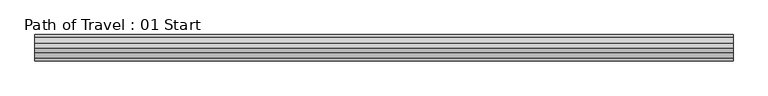
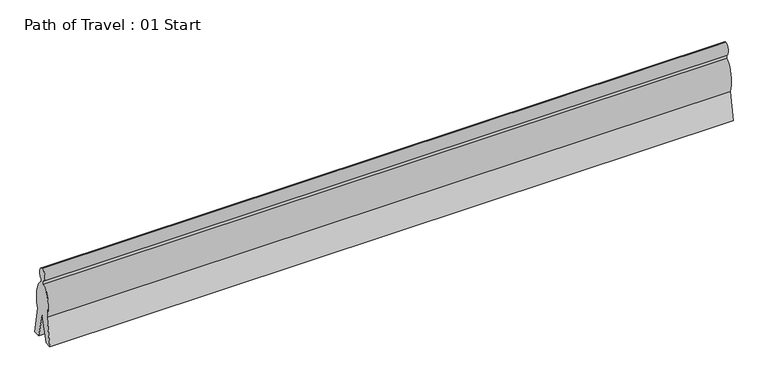
"""IFC4 building model written with IfcOpenShell, lengths in millimetres: proxy geometry, Path of Travel : 01 Start."""

import ifcopenshell
import ifcopenshell.guid

model = None  # the IFC model being written
_history = None  # IfcOwnerHistory: only IFC2X3 demands one
_inside = {}  # id of a spatial element -> (the spatial element, [elements in it])
_under = {}  # id of a project, library or spatial element -> (it, [spatial elements below it])
_declared = {}  # id of a project -> (the project, [libraries it declares])
_typed = {}  # id of a type object -> (the type object, [elements of that type])
_made_of = {}  # id of a material, layer set ... -> (it, [elements and type objects made of it])


def new_model(schema):
    """Start an empty IFC model of exactly this schema.

    Asked for "IFC4X3", IfcOpenShell would pick the latest addendum, in which some entities
    have other attributes; the version numbers below select the first issue.
    IFC2X3 requires an IfcOwnerHistory on every rooted entity: one is made here for all.
    """
    global model, _history
    if schema == "IFC4X3":
        model = ifcopenshell.file(schema_version=(4, 3, 0, 0))
    else:
        model = ifcopenshell.file(schema=schema)
    _inside.clear()
    _under.clear()
    _declared.clear()
    _typed.clear()
    _made_of.clear()
    _history = None
    if model.schema == "IFC2X3":
        org = make("IfcOrganization", Name="unknown")
        user = make(
            "IfcPersonAndOrganization",
            ThePerson=make("IfcPerson", FamilyName="unknown"),
            TheOrganization=org,
        )
        app = make(
            "IfcApplication",
            ApplicationDeveloper=org,
            Version="unknown",
            ApplicationFullName="unknown",
            ApplicationIdentifier="unknown",
        )
        _history = make(
            "IfcOwnerHistory",
            OwningUser=user,
            OwningApplication=app,
            ChangeAction="ADDED",
            CreationDate=0,
        )
    return model


def make(cls, **values):
    """One entity of the class cls with the attributes given. An attribute that is None is left unset."""
    return model.create_entity(
        cls, **{name: value for name, value in values.items() if value is not None}
    )


def rooted(cls, **values):
    """An entity with a GlobalId (a new one), such as an element, a storey or a relation."""
    return make(cls, GlobalId=ifcopenshell.guid.new(), OwnerHistory=_history, **values)


def si_unit(unit_type, name, prefix=None):
    """IfcSIUnit, for example si_unit("LENGTHUNIT", "METRE", prefix="MILLI")."""
    return make("IfcSIUnit", UnitType=unit_type, Prefix=prefix, Name=name)


def assignment(units):
    """IfcUnitAssignment: the units of a project."""
    return None if units is None else make("IfcUnitAssignment", Units=units)


def point(xyz):
    """IfcCartesianPoint."""
    return None if xyz is None else make("IfcCartesianPoint", Coordinates=xyz)


def direction(xyz):
    """IfcDirection."""
    return None if xyz is None else make("IfcDirection", DirectionRatios=xyz)


def frame(location, z_axis=None, x_axis=None):
    """IfcAxis2Placement3D, a coordinate frame: its origin and axes. An axis left out is left unset."""
    return make(
        "IfcAxis2Placement3D",
        Location=point(location),
        Axis=direction(z_axis),
        RefDirection=direction(x_axis),
    )


def origin():
    """The frame at (0, 0, 0) with its axes left unset."""
    return frame((0.0, 0.0, 0.0))


def place(relative_to, where):
    """IfcLocalPlacement: puts the frame where relative to a parent placement (None: the world)."""
    return make(
        "IfcLocalPlacement", PlacementRelTo=relative_to, RelativePlacement=where
    )


def context(
    kind, dimensions, precision=None, world=None, true_north=None, identifier=None
):
    """IfcGeometricRepresentationContext, for example the 3D "Model" context."""
    return make(
        "IfcGeometricRepresentationContext",
        ContextIdentifier=identifier,
        ContextType=kind,
        CoordinateSpaceDimension=dimensions,
        Precision=precision,
        WorldCoordinateSystem=world,
        TrueNorth=true_north,
    )


def project(units=None, contexts=None):
    """IfcProject with its units and contexts."""
    return rooted(
        "IfcProject",
        Name="project",
        RepresentationContexts=contexts,
        UnitsInContext=assignment(units),
    )


def spatial(cls, under=None, at=None, **own):
    """A site, building, storey or space (cls), placed at a placement, below another one or the project."""
    s = rooted(cls, ObjectPlacement=at, **own)
    if under is not None:
        _under.setdefault(under.id(), (under, []))[1].append(s)
    return s


def ellipse_curve(where, semi_axis1, semi_axis2):
    """IfcEllipse in the frame where."""
    return make(
        "IfcEllipse", Position=where, SemiAxis1=semi_axis1, SemiAxis2=semi_axis2
    )


def trimmed(basis, trim1, trim2, sense, master):
    """IfcTrimmedCurve: the piece of a basis curve between two trims."""
    return make(
        "IfcTrimmedCurve",
        BasisCurve=basis,
        Trim1=trim1,
        Trim2=trim2,
        SenseAgreement=sense,
        MasterRepresentation=master,
    )


def shape(context_of_items, identifier, shape_type, items):
    """IfcShapeRepresentation: the items that make up one representation, for example the "Body"."""
    return make(
        "IfcShapeRepresentation",
        ContextOfItems=context_of_items,
        RepresentationIdentifier=identifier,
        RepresentationType=shape_type,
        Items=items,
    )


def source(mapping_origin, context_of_items, identifier, shape_type, items):
    """IfcRepresentationMap: a shape defined once, which mapped items show again and again."""
    return make(
        "IfcRepresentationMap",
        MappingOrigin=mapping_origin,
        MappedRepresentation=shape(context_of_items, identifier, shape_type, items),
    )


def transform(
    local_origin,
    x_axis=None,
    y_axis=None,
    z_axis=None,
    scale=None,
    scale2=None,
    scale3=None,
    uniform=True,
):
    """IfcCartesianTransformationOperator3D, or its non-uniform kind. x_axis, y_axis, z_axis: its Axis1, 2, 3."""
    if uniform:
        return make(
            "IfcCartesianTransformationOperator3D",
            Axis1=direction(x_axis),
            Axis2=direction(y_axis),
            LocalOrigin=point(local_origin),
            Scale=scale,
            Axis3=direction(z_axis),
        )
    return make(
        "IfcCartesianTransformationOperator3DnonUniform",
        Axis1=direction(x_axis),
        Axis2=direction(y_axis),
        LocalOrigin=point(local_origin),
        Scale=scale,
        Axis3=direction(z_axis),
        Scale2=scale2,
        Scale3=scale3,
    )


def mapped(mapping_source, mapping_target):
    """IfcMappedItem: shows the shape of a source again, moved by a transform."""
    return make(
        "IfcMappedItem", MappingSource=mapping_source, MappingTarget=mapping_target
    )


def made_of(thing, what):
    """Note that an element or type object is made of a material, layer set ...; save() writes the relation."""
    if what is not None:
        _made_of.setdefault(what.id(), (what, []))[1].append(thing)
    return thing


def element(
    cls,
    number,
    at=None,
    inside=None,
    cuts=None,
    type_object=None,
    material=None,
    context=None,
    identifier="Body",
    shape_type=None,
    held_by="IfcProductDefinitionShape",
    body=None,
    shapes=None,
    **own,
):
    """One element of the class cls, such as IfcWall. Its Tag is "e" and its number.

    at: its placement. inside: the storey or other place that contains it. cuts: it is an
    opening in that element (IfcRelVoidsElement). A single representation is given by context,
    identifier, shape_type and body (its items); several are given by shapes. held_by: the class
    of the entity that holds the representations. save() writes the other relations.
    """
    e = rooted(cls, Tag="e%d" % number, ObjectPlacement=at, **own)
    if body is not None:
        shapes = [shape(context, identifier, shape_type, body)]
    if shapes is not None:
        e.Representation = make(held_by, Representations=shapes)
    if inside is not None:
        _inside.setdefault(inside.id(), (inside, []))[1].append(e)
    if cuts is not None:
        rooted(
            "IfcRelVoidsElement", RelatingBuildingElement=cuts, RelatedOpeningElement=e
        )
    if type_object is not None:
        _typed.setdefault(type_object.id(), (type_object, []))[1].append(e)
    return made_of(e, material)


def aggregate(whole, parts):
    """IfcRelAggregates: a whole, such as a stair, and the parts it consists of."""
    return rooted("IfcRelAggregates", RelatingObject=whole, RelatedObjects=parts)


def save(model, path):
    """Write the relations noted so far, then the file.

    IfcRelAggregates (storeys below a building ...), IfcRelContainedInSpatialStructure (elements
    in a storey), IfcRelDefinesByType, IfcRelAssociatesMaterial and IfcRelDeclares: one each for
    every whole, place, type object, material and project.
    """
    for whole, parts in _under.values():
        aggregate(whole, parts)
    for where, things in _inside.values():
        rooted(
            "IfcRelContainedInSpatialStructure",
            RelatedElements=things,
            RelatingStructure=where,
        )
    for kind, things in _typed.values():
        rooted("IfcRelDefinesByType", RelatedObjects=things, RelatingType=kind)
    for what, things in _made_of.values():
        rooted("IfcRelAssociatesMaterial", RelatedObjects=things, RelatingMaterial=what)
    for by, libraries in _declared.values():
        rooted("IfcRelDeclares", RelatingContext=by, RelatedDefinitions=libraries)
    model.write(path)


def plane_surface(at):
    """IfcPlane: the flat surface through the origin of the frame at, square to its z axis."""
    return make("IfcPlane", Position=at)


def extruded_surface(curve, direction_of_extrusion, depth):
    """IfcSurfaceOfLinearExtrusion: the curve pushed along a direction by depth."""
    return make(
        "IfcSurfaceOfLinearExtrusion",
        SweptCurve=make("IfcArbitraryOpenProfileDef", ProfileType="CURVE", Curve=curve),
        ExtrudedDirection=direction(direction_of_extrusion),
        Depth=depth,
    )


def advanced_brep(points, edges, surfaces, faces):
    """IfcAdvancedBrep: a solid bounded by faces that lie on surfaces and meet in shared edges.

    An edge is (start, end): straight between two places in points (the first is 0);
    or (start, end, curve); or (start, end, curve, False) where it runs against its curve.
    A face is (place in surfaces, loops), or (place, loops, False) where it looks against
    its surface's normal. A loop lists edges by number (the first is 1), with a minus sign
    where the edge is run from its end to its start. The first loop is the outer one.
    """
    corners = [point(p) for p in points]
    vertices = [make("IfcVertexPoint", VertexGeometry=c) for c in corners]
    made = []
    for start, end, *more in edges:
        made.append(
            make(
                "IfcEdgeCurve",
                EdgeStart=vertices[start],
                EdgeEnd=vertices[end],
                EdgeGeometry=more[0] if more else make("IfcPolyline", Points=[corners[start], corners[end]]),
                SameSense=more[1] if len(more) > 1 else True,
            )
        )
    hull = []
    for where, loops, *sense in faces:
        bounds = []
        for j, loop in enumerate(loops):
            ring = [make("IfcOrientedEdge", EdgeElement=made[abs(k) - 1], Orientation=k > 0) for k in loop]
            bounds.append(
                make(
                    "IfcFaceOuterBound" if j == 0 else "IfcFaceBound",
                    Bound=make("IfcEdgeLoop", EdgeList=ring),
                    Orientation=True,
                )
            )
        hull.append(make("IfcAdvancedFace", Bounds=bounds, FaceSurface=surfaces[where], SameSense=sense[0] if sense else True))
    return make("IfcAdvancedBrep", Outer=make("IfcClosedShell", CfsFaces=hull))


def path_of_travel_01_start_b18a8849(model_context):
    return source(origin(), model_context, "Body", "AdvancedBrep", [
        advanced_brep(
        [(227.5554837, 0.0, 1727.2), (227.5554837, 42.9018657, 1436.6534209), (227.5554837, 42.9018657, 1363.4763406), (227.5554837, 184.1186263, 643.4144547), (227.5554837, 297.5699544, 0.0), (227.5554837, 145.6574193, 0.0), (227.5554837, 0.0, 584.2), (227.5554837, -145.6574193, 0.0), (227.5554837, -297.5699544, 0.0), (227.5554837, -184.1186263, 643.4144547), (227.5554837, -42.9018657, 1363.4763406), (227.5554837, -42.9018657, 1436.6534209), (15924.7554837, 0.0, 1727.2), (15924.7554837, -42.9018657, 1436.6534209), (15924.7554837, -42.9018657, 1363.4763406), (15924.7554837, -184.1186263, 643.4144547), (15924.7554837, -297.5699544, 0.0), (15924.7554837, -145.6574193, 0.0), (15924.7554837, 0.0, 584.2), (15924.7554837, 145.6574193, 0.0), (15924.7554837, 297.5699544, 0.0), (15924.7554837, 184.1186263, 643.4144547), (15924.7554837, 42.9018657, 1363.4763406), (15924.7554837, 42.9018657, 1436.6534209)],
        [
            (0, 1, ellipse_curve(frame((227.5554837, 0.0, 1574.8), z_axis=(-1.0, 0.0, 0.0), x_axis=(0.0, 0.0, 1.0)), 152.4, 101.6)),
            (1, 2),
            (2, 3, ellipse_curve(frame((227.5554837, 0.0, 914.4), z_axis=(-1.0, 0.0, 0.0), x_axis=(0.0, 0.0, -1.0)), 457.2, 228.6)),
            (3, 4),
            (4, 5),
            (5, 6),
            (6, 7),
            (7, 8),
            (8, 9),
            (9, 10, ellipse_curve(frame((227.5554837, 0.0, 914.4), z_axis=(-1.0, 0.0, 0.0), x_axis=(0.0, 0.0, -1.0)), 457.2, 228.6)),
            (10, 11),
            (11, 0, ellipse_curve(frame((227.5554837, 0.0, 1574.8), z_axis=(-1.0, 0.0, 0.0), x_axis=(0.0, 0.0, 1.0)), 152.4, 101.6)),
            (12, 13, ellipse_curve(frame((15924.7554837, 0.0, 1574.8), z_axis=(1.0, 0.0, 0.0), x_axis=(0.0, 0.0, 1.0)), 152.4, 101.6)),
            (13, 14),
            (14, 15, ellipse_curve(frame((15924.7554837, 0.0, 914.4), z_axis=(1.0, 0.0, 0.0), x_axis=(0.0, 0.0, -1.0)), 457.2, 228.6)),
            (15, 16),
            (16, 17),
            (17, 18),
            (18, 19),
            (19, 20),
            (20, 21),
            (21, 22, ellipse_curve(frame((15924.7554837, 0.0, 914.4), z_axis=(1.0, 0.0, 0.0), x_axis=(0.0, 0.0, -1.0)), 457.2, 228.6)),
            (22, 23),
            (23, 12, ellipse_curve(frame((15924.7554837, 0.0, 1574.8), z_axis=(1.0, 0.0, 0.0), x_axis=(0.0, 0.0, 1.0)), 152.4, 101.6)),
            (0, 12),
            (23, 1),
            (22, 2),
            (21, 3),
            (20, 4),
            (19, 5),
            (18, 6),
            (17, 7),
            (16, 8),
            (15, 9),
            (14, 10),
            (13, 11),
        ],
        [
            plane_surface(frame((227.5554837, 0.0, 0.0), z_axis=(-1.0, 0.0, 0.0), x_axis=(0.0, 0.0, 1.0))),
            plane_surface(frame((15924.7554837, 0.0, 0.0), z_axis=(1.0, 0.0, 0.0), x_axis=(0.0, 0.0, 1.0))),
            extruded_surface(trimmed(ellipse_curve(frame((15924.7554837, 0.0, 1574.8), z_axis=(-1.0, 0.0, 0.0), x_axis=(0.0, 0.0, 1.0)), 152.4, 101.6), [point((15924.7554837, 0.0, 1727.2))], [point((15924.7554837, 42.9018657, 1436.6534209))], True, "CARTESIAN"), (-15697.2, 0.0, 0.0), 15697.2),
            plane_surface(frame((227.5554837, 42.9018657, 1436.6534209), z_axis=(0.0, 1.0, 0.0), x_axis=(1.0, 0.0, 0.0))),
            extruded_surface(trimmed(ellipse_curve(frame((15924.7554837, 0.0, 914.4), z_axis=(-1.0, 0.0, 0.0), x_axis=(0.0, 0.0, -1.0)), 457.2, 228.6), [point((15924.7554837, 42.9018657, 1363.4763406))], [point((15924.7554837, 184.1186263, 643.4144547))], True, "CARTESIAN"), (-15697.2, 0.0, 0.0), 15697.2),
            plane_surface(frame((227.5554837, 184.1186263, 643.4144547), z_axis=(0.0, 0.9848077530122078, 0.17364817766693205), x_axis=(1.0, 0.0, 0.0))),
            plane_surface(frame((227.5554837, 297.5699544, 0.0), z_axis=(0.0, 0.0, -1.0), x_axis=(1.0, 0.0, 0.0))),
            plane_surface(frame((227.5554837, 145.6574193, 0.0), z_axis=(0.0, -0.9702957262760199, -0.2419218955995739), x_axis=(1.0, 0.0, 0.0))),
            plane_surface(frame((227.5554837, 0.0, 584.2), z_axis=(0.0, 0.9702957262759961, -0.24192189559966923), x_axis=(1.0, 0.0, 0.0))),
            plane_surface(frame((227.5554837, -145.6574193, 0.0), z_axis=(0.0, 0.0, -1.0), x_axis=(1.0, 0.0, 0.0))),
            plane_surface(frame((227.5554837, -297.5699544, 0.0), z_axis=(0.0, -0.984807753012208, 0.17364817766693066), x_axis=(1.0, 0.0, 0.0))),
            extruded_surface(trimmed(ellipse_curve(frame((15924.7554837, 0.0, 914.4), z_axis=(-1.0, 0.0, 0.0), x_axis=(0.0, 0.0, -1.0)), 457.2, 228.6), [point((15924.7554837, -184.1186263, 643.4144547))], [point((15924.7554837, -42.9018657, 1363.4763406))], True, "CARTESIAN"), (-15697.2, 0.0, 0.0), 15697.2),
            plane_surface(frame((227.5554837, -42.9018657, 1363.4763406), z_axis=(0.0, -1.0, 0.0), x_axis=(1.0, 0.0, 0.0))),
            extruded_surface(trimmed(ellipse_curve(frame((15924.7554837, 0.0, 1574.8), z_axis=(-1.0, 0.0, 0.0), x_axis=(0.0, 0.0, 1.0)), 152.4, 101.6), [point((15924.7554837, -42.9018657, 1436.6534209))], [point((15924.7554837, 0.0, 1727.2))], True, "CARTESIAN"), (-15697.2, 0.0, 0.0), 15697.2),
        ],
        [
            (0, [[1, 2, 3, 4, 5, 6, 7, 8, 9, 10, 11, 12]]),
            (1, [[13, 14, 15, 16, 17, 18, 19, 20, 21, 22, 23, 24]]),
            (2, [[-1, 25, -24, 26]]),
            (3, [[-2, -26, -23, 27]]),
            (4, [[-3, -27, -22, 28]]),
            (5, [[-4, -28, -21, 29]]),
            (6, [[-5, -29, -20, 30]]),
            (7, [[-6, -30, -19, 31]]),
            (8, [[-7, -31, -18, 32]]),
            (9, [[-8, -32, -17, 33]]),
            (10, [[-9, -33, -16, 34]]),
            (11, [[-10, -34, -15, 35]]),
            (12, [[-11, -35, -14, 36]]),
            (13, [[-12, -36, -13, -25]]),
        ],
    ),
    ])


if __name__ == "__main__":
    model = new_model("IFC4")
    model_context = context("Model", 3, world=origin())
    ifc_project = project(units=[si_unit("LENGTHUNIT", "METRE", prefix="MILLI")], contexts=[model_context])
    site = spatial("IfcSite", under=ifc_project)
    building = spatial("IfcBuilding", under=site)
    placement = place(None, origin())
    path_of_travel_01_start_shape = path_of_travel_01_start_b18a8849(model_context)
    element("IfcBuildingElementProxy", 1, Name="Path of Travel : 01 Start", ObjectType="Path of Travel : 01 Start", at=placement, inside=building, context=model_context, shape_type="MappedRepresentation", body=[
        mapped(path_of_travel_01_start_shape, transform((0.0, 0.0, 0.0), x_axis=(1.0, 0.0, 0.0), y_axis=(0.0, 1.0, 0.0), z_axis=(0.0, 0.0, 1.0))),
    ])
    save(model, "model.ifc")

# Revit data of these elements
# Type "Path of Travel : 01 Start"
#   Path of Egress [instance default] = 4' - 0"
#   built-in parameter 1001306 [instance default] = 4 (stored number, unit not read)
#   Dot at Start = yes
#   Arrow in Middle = yes
#   Arrow at End = no
#   Egress Path = none
# Element 1 (IfcBuildingElementProxy, "Path of Travel : 01 Start")
#   Path of Egress = 51' - 6"
#   built-in parameter 1001306 = 51.5 (stored number, unit not read)
#   Materials on its faces: "Egress Path Solid"
# Materials
#   "Egress Path Solid": class "Unassigned", colour RGB 255 128 64, transparency 0.75, Comments = "Rendering appearance not upgraded "
